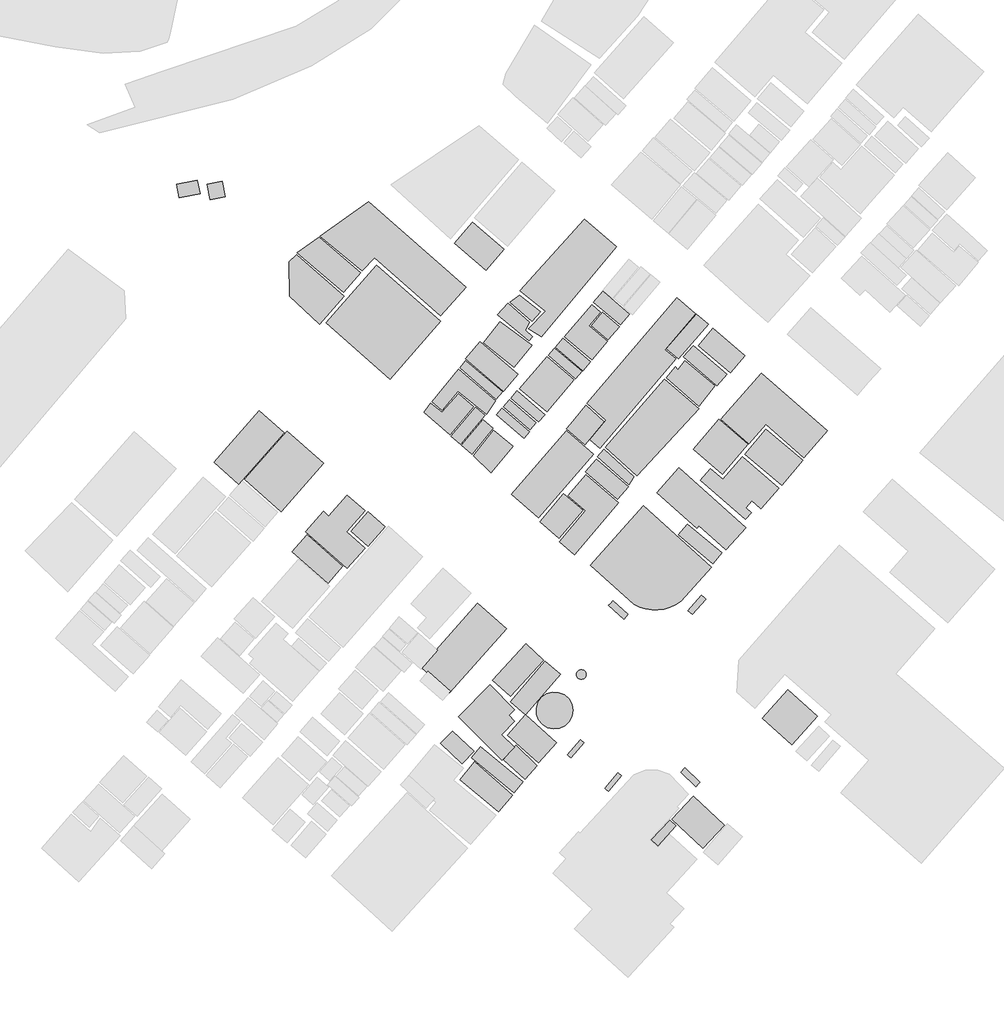
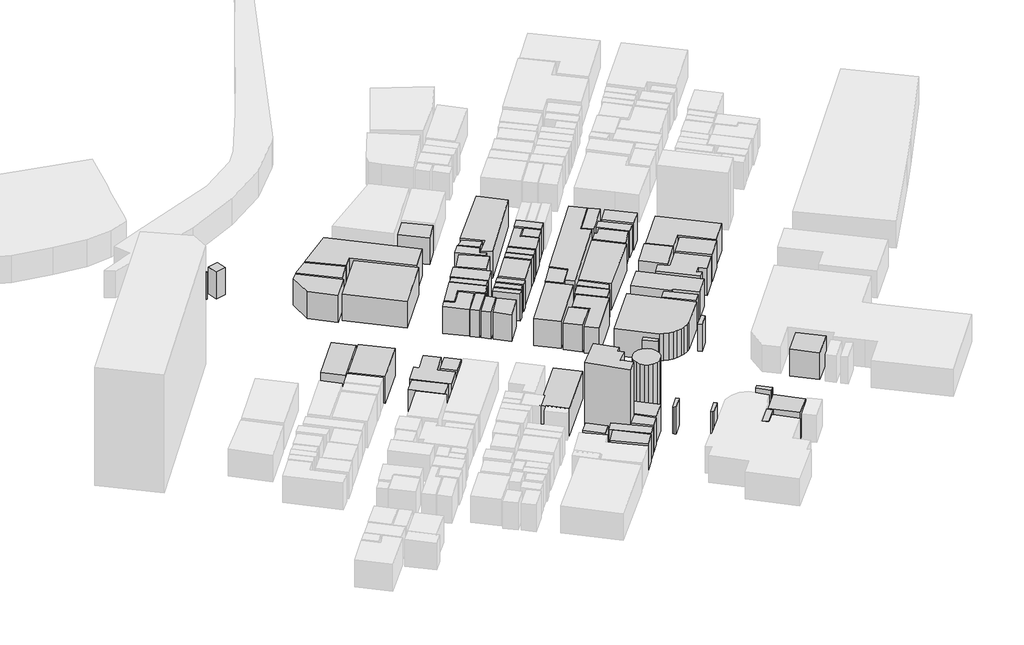
# Not in any storey, part 2 of 3: 70 proxies.
"""IFC4 building model written with IfcOpenShell, lengths in millimetres."""

from ifc_helpers import new_model, si_unit, origin, origin_with_axes, place, context, project, spatial, polyline, outline, extrude, element, save

model = new_model("IFC4")

# Units and contexts
model_context = context("Model", 3, world=origin())
ifc_project = project(units=[si_unit("LENGTHUNIT", "METRE", prefix="MILLI")], contexts=[model_context])

# Site, building
site = spatial("IfcSite", under=ifc_project)
building = spatial("IfcBuilding", under=site)

# Proxies
placement = place(None, origin())
element("IfcBuildingElementProxy", 1, Name="Mass", at=placement, inside=building, context=model_context, shape_type="SweptSolid", body=[
    extrude(outline(polyline([(170698.7323915, 46624.0327425), (171096.1893538, 44511.3291361), (170789.0635192, 42387.5060369), (169804.4542245, 40486.0727911), (168268.8250515, 38984.9412821), (166326.7058014, 38073.1428832), (164194.8911837, 37828.5140449), (162099.2090151, 38284.4132439), (160265.4871197, 39385.2430179), (158883.4208628, 41030.9279318), (158097.5400505, 43054.6755966), (158016.2420351, 45234.096159), (158657.593041, 47313.4412879), (159931.2619458, 49070.3211289), (161719.8182773, 50315.7043068), (163815.500446, 50905.0374178), (165983.4475152, 50782.7229987), (167997.8316659, 49959.8805414), (169623.7919691, 48514.3464955), (170698.7323915, 46624.0327425)])), origin_with_axes(), (0.0, 0.0, 1.0), 35000.0),
])
element("IfcBuildingElementProxy", 2, Name="Mass", at=placement, inside=building, context=model_context, shape_type="SweptSolid", body=[
    extrude(outline(polyline([(130374.9168956, 42153.9966913), (141485.6456275, 53473.6402233), (150256.798147, 44678.1215256), (148287.5795602, 42676.6128464), (150310.9968231, 40486.0727911), (145677.0099623, 35793.6468872), (150175.5001316, 31245.7743872), (145848.6391053, 26586.7069609), (130374.9168956, 42153.9966913)])), origin_with_axes(), (0.0, 0.0, 1.0), 45000.0),
])
element("IfcBuildingElementProxy", 3, Name="Mass", at=placement, inside=building, context=model_context, shape_type="SweptSolid", body=[
    extrude(outline(polyline([(208574.5743203, 165836.1135976), (210995.448548, 168927.3325589), (221636.4554144, 160031.7384269), (215927.5281312, 152781.8292102), (204419.3424371, 162933.9260122), (207608.0312501, 166803.5094596), (208574.5743203, 165836.1135976)])), origin_with_axes(), (0.0, 0.0, 1.0), 15000.0),
])
element("IfcBuildingElementProxy", 4, Name="Mass", at=placement, inside=building, context=model_context, shape_type="SweptSolid", body=[
    extrude(outline(polyline([(177934.2557355, 188964.6583397), (180978.4147472, 186362.6970567), (176868.3484279, 181547.9567328), (183462.5207633, 175921.4934444), (177780.6928194, 169283.1563236), (168151.3945845, 177511.5808958), (177934.2557355, 188964.6583397)])), origin_with_axes(), (0.0, 0.0, 1.0), 15000.0),
])
element("IfcBuildingElementProxy", 5, Name="Mass", at=placement, inside=building, context=model_context, shape_type="SweptSolid", body=[
    extrude(outline(polyline([(164809.1428529, 173875.5067947), (167519.0766882, 177044.562204), (177310.970954, 168671.5842278), (174601.0371162, 165502.5288177), (164809.1428529, 173875.5067947)])), origin_with_axes(), (0.0, 0.0, 1.0), 15000.0),
])
element("IfcBuildingElementProxy", 6, Name="Mass", at=placement, inside=building, context=model_context, shape_type="SweptSolid", body=[
    extrude(outline(polyline([(146282.2285192, 152626.1563127), (148432.1093639, 155139.161655), (157980.1095835, 146988.5735315), (155830.2287387, 144475.5681892), (146282.2285192, 152626.1563127)])), origin_with_axes(), (0.0, 0.0, 1.0), 15000.0),
])
element("IfcBuildingElementProxy", 7, Name="Mass", at=placement, inside=building, context=model_context, shape_type="SweptSolid", body=[
    extrude(outline(polyline([(186524.7459996, 209546.839262), (159931.2619458, 177633.895315), (155288.2419727, 180347.0515252), (161286.2288635, 186629.5648806), (152289.2485248, 193979.5495315), (175215.2887854, 219409.8292553), (186524.7459996, 209546.839262)])), origin_with_axes(), (0.0, 0.0, 1.0), 15000.0),
])
element("IfcBuildingElementProxy", 8, Name="Mass", at=placement, inside=building, context=model_context, shape_type="SweptSolid", body=[
    extrude(outline(polyline([(247760.2176028, 51805.7163239), (258292.8271145, 42287.4306033), (249151.3169721, 32168.6922789), (238618.7074578, 41686.9779995), (247760.2176028, 51805.7163239)])), origin_with_axes(), (0.0, 0.0, 1.0), 15000.0),
])
element("IfcBuildingElementProxy", 9, Name="Mass", at=placement, inside=building, context=model_context, shape_type="SweptSolid", body=[
    extrude(outline(polyline([(145125.990084, 182937.8933163), (156489.6459718, 174520.4373689), (150148.4007948, 166681.1950405), (139254.4667699, 175421.116275), (145125.990084, 182937.8933163)])), origin_with_axes(), (0.0, 0.0, 1.0), 15000.0),
])
element("IfcBuildingElementProxy", 10, Name="Mass", at=placement, inside=building, context=model_context, shape_type="SweptSolid", body=[
    extrude(outline(polyline([(139028.6389507, 148000.447364), (142551.5529376, 144864.7504331), (135026.9699836, 135657.8105068), (131350.4930781, 138860.2243936), (139028.6389507, 148000.447364)])), origin_with_axes(), (0.0, 0.0, 1.0), 15000.0),
])
element("IfcBuildingElementProxy", 11, Name="Mass", at=placement, inside=building, context=model_context, shape_type="SweptSolid", body=[
    extrude(outline(polyline([(215792.0314397, 174387.0034569), (221031.2368575, 180524.9634075), (232394.8927479, 170817.6463118), (227155.6873275, 164679.6863612), (215792.0314397, 174387.0034569)])), origin_with_axes(), (0.0, 0.0, 1.0), 15000.0),
])
element("IfcBuildingElementProxy", 12, Name="Mass", at=placement, inside=building, context=model_context, shape_type="SweptSolid", body=[
    extrude(outline(polyline([(203868.3225562, 173008.1863662), (207725.4617171, 169716.8165378), (180707.4213617, 137803.8725908), (177220.6398263, 140939.5695225), (182839.2359819, 147878.1329448), (176109.5669524, 153916.0174618), (208177.117358, 191455.4246972), (214798.3890328, 185795.6029305), (203868.3225562, 173008.1863662)])), origin_with_axes(), (0.0, 0.0, 1.0), 15000.0),
])
element("IfcBuildingElementProxy", 13, Name="Mass", at=placement, inside=building, context=model_context, shape_type="SweptSolid", body=[
    extrude(outline(polyline([(138025.9634289, 175721.3425765), (151422.0696971, 164268.2651325), (146246.0960676, 158219.2611227), (132849.9898021, 169672.3385674), (138025.9634289, 175721.3425765)])), origin_with_axes(), (0.0, 0.0, 1.0), 15000.0),
])
element("IfcBuildingElementProxy", 14, Name="Mass", at=placement, inside=building, context=model_context, shape_type="SweptSolid", body=[
    extrude(outline(polyline([(162334.0699465, 170951.0802238), (164502.0170183, 173486.3245509), (174230.6794932, 165180.0635306), (172053.6993091, 162633.6997107), (162334.0699465, 170951.0802238)])), origin_with_axes(), (0.0, 0.0, 1.0), 15000.0),
])
element("IfcBuildingElementProxy", 15, Name="Mass", at=placement, inside=building, context=model_context, shape_type="SweptSolid", body=[
    extrude(outline(polyline([(187355.7923757, 118344.7604281), (171556.8781069, 99930.8805755), (166218.3084467, 104512.1115531), (175630.8119747, 115475.9313204), (169334.732359, 120880.0047552), (175721.1431024, 128318.9453478), (187355.7923757, 118344.7604281)])), origin_with_axes(), (0.0, 0.0, 1.0), 15000.0),
])
element("IfcBuildingElementProxy", 16, Name="Mass", at=placement, inside=building, context=model_context, shape_type="SweptSolid", body=[
    extrude(outline(polyline([(168792.745593, 144742.4360131), (170156.7456229, 146410.3599133), (175648.8781992, 153137.6529749), (182152.7194095, 147299.9193266), (175323.6861401, 139104.8532327), (168792.745593, 144742.4360131)])), origin_with_axes(), (0.0, 0.0, 1.0), 15000.0),
])
element("IfcBuildingElementProxy", 17, Name="Mass", at=placement, inside=building, context=model_context, shape_type="SweptSolid", body=[
    extrude(outline(polyline([(144186.5463531, 185328.5842386), (147953.3543863, 189565.1109435), (155676.6658227, 182782.2204187), (154159.1028717, 179813.3158774), (156715.4737935, 177600.5368366), (155333.4075365, 176043.8078635), (144186.5463531, 185328.5842386)])), origin_with_axes(), (0.0, 0.0, 1.0), 15000.0),
])
element("IfcBuildingElementProxy", 18, Name="Mass", at=placement, inside=building, context=model_context, shape_type="SweptSolid", body=[
    extrude(outline(polyline([(148956.0299055, 155661.77781), (151160.1094263, 158241.5001083), (161060.4010443, 149779.5661905), (158856.3215234, 147199.8438922), (148956.0299055, 155661.77781)])), origin_with_axes(), (0.0, 0.0, 1.0), 15000.0),
])
element("IfcBuildingElementProxy", 19, Name="Mass", at=placement, inside=building, context=model_context, shape_type="SweptSolid", body=[
    extrude(outline(polyline([(182649.5406117, 138148.5768635), (203660.5609616, 162455.7878276), (216017.8592589, 151903.3892898), (193940.9315989, 128085.4360023), (182649.5406117, 138148.5768635)])), origin_with_axes(), (0.0, 0.0, 1.0), 15000.0),
])
element("IfcBuildingElementProxy", 20, Name="Mass", at=placement, inside=building, context=model_context, shape_type="SweptSolid", body=[
    extrude(outline(polyline([(143852.3211792, 149790.6856833), (145812.5066538, 152081.3011721), (155622.4671441, 143697.2037031), (153662.2816695, 141395.4687215), (143852.3211792, 149790.6856833)])), origin_with_axes(), (0.0, 0.0, 1.0), 15000.0),
])
element("IfcBuildingElementProxy", 21, Name="Mass", at=placement, inside=building, context=model_context, shape_type="SweptSolid", body=[
    extrude(outline(polyline([(130230.3870919, 157296.3432318), (135695.4203289, 152537.2003711), (127195.2611949, 142629.7324075), (117945.3536977, 150635.7671254), (120375.2610377, 153838.1810131), (124494.3604693, 150591.289155), (130230.3870919, 157296.3432318)])), origin_with_axes(), (0.0, 0.0, 1.0), 15000.0),
])
element("IfcBuildingElementProxy", 22, Name="Mass", at=placement, inside=building, context=model_context, shape_type="SweptSolid", body=[
    extrude(outline(polyline([(120881.1153548, 154405.2751393), (130338.7844466, 166025.1449735), (143545.1953446, 154672.1429632), (140257.1422891, 150001.956044), (130149.0890765, 158152.5441667), (124367.8968926, 151447.4900899), (120881.1153548, 154405.2751393)])), origin_with_axes(), (0.0, 0.0, 1.0), 15000.0),
])
element("IfcBuildingElementProxy", 23, Name="Mass", at=placement, inside=building, context=model_context, shape_type="SweptSolid", body=[
    extrude(outline(polyline([(177654.2292402, 181525.7177472), (181682.9975441, 186251.5021295), (187644.8519858, 181158.7744897), (183607.0505671, 176444.1096002), (177654.2292402, 181525.7177472)])), origin_with_axes(), (0.0, 0.0, 1.0), 15000.0),
])
element("IfcBuildingElementProxy", 24, Name="Mass", at=placement, inside=building, context=model_context, shape_type="SweptSolid", body=[
    extrude(outline(polyline([(142849.64566, 144219.8198581), (149778.0431693, 138471.0421506), (141955.3674929, 129052.8318643), (135659.2878798, 135157.4333365), (142849.64566, 144219.8198581)])), origin_with_axes(), (0.0, 0.0, 1.0), 15000.0),
])
element("IfcBuildingElementProxy", 25, Name="Mass", at=placement, inside=building, context=model_context, shape_type="SweptSolid", body=[
    extrude(outline(polyline([(231563.8463692, 134768.2510935), (244463.1314351, 123582.0414727), (238121.8862556, 116276.5347921), (234933.1974401, 119034.1689735), (232765.2503708, 116532.283124), (234617.0384932, 114919.9566878), (232530.3894394, 112518.1462718), (216550.8129127, 126384.1536245), (220164.0580298, 130542.8438806), (224581.2501837, 126717.7384044), (231563.8463692, 134768.2510935)])), origin_with_axes(), (0.0, 0.0, 1.0), 15000.0),
])
element("IfcBuildingElementProxy", 26, Name="Mass", at=placement, inside=building, context=model_context, shape_type="SweptSolid", body=[
    extrude(outline(polyline([(192902.1236281, 82150.8118051), (177265.8053902, 96139.1335769), (196163.0773468, 117277.2891325), (220516.3494282, 95494.2030027), (209559.183615, 83240.5220863), (207707.3954926, 82039.6168787), (205693.0113393, 81116.6989878), (203579.2629461, 80505.1268912), (201393.2496524, 80193.7810962), (199180.1370193, 80216.0200818), (197003.1568352, 80549.6048616), (194889.4084421, 81205.6549286), (192902.1236281, 82150.8118051)])), origin_with_axes(), (0.0, 0.0, 1.0), 15000.0),
])
element("IfcBuildingElementProxy", 27, Name="Mass", at=placement, inside=building, context=model_context, shape_type="SweptSolid", body=[
    extrude(outline(polyline([(200959.6602385, 121969.7150364), (208881.7001549, 130854.1896757), (232729.1179192, 109571.4807161), (225656.1906061, 101654.4019389), (216053.9917105, 110216.4112902), (215204.8791073, 109260.134921), (200959.6602385, 121969.7150364)])), origin_with_axes(), (0.0, 0.0, 1.0), 15000.0),
])
element("IfcBuildingElementProxy", 28, Name="Mass", at=placement, inside=building, context=model_context, shape_type="SweptSolid", body=[
    extrude(outline(polyline([(175567.5801838, 129464.2530922), (179424.7193472, 133923.1696506), (190842.5739136, 124060.1796573), (186994.4678651, 119601.2630989), (175567.5801838, 129464.2530922)])), origin_with_axes(), (0.0, 0.0, 1.0), 15000.0),
])
element("IfcBuildingElementProxy", 29, Name="Mass", at=placement, inside=building, context=model_context, shape_type="SweptSolid", body=[
    extrude(outline(polyline([(161204.930848, 61913.3351563), (166579.6329599, 57298.7457003), (154249.4340019, 42943.4806703), (148874.73189, 47558.0701262), (161204.930848, 61913.3351563)])), origin_with_axes(), (0.0, 0.0, 1.0), 15000.0),
])
element("IfcBuildingElementProxy", 30, Name="Mass", at=placement, inside=building, context=model_context, shape_type="SweptSolid", body=[
    extrude(outline(polyline([(130916.9036642, 19659.2630314), (135975.4468267, 26086.3297907), (149488.9835592, 14199.5921325), (144493.6721877, 8317.380513), (130916.9036642, 19659.2630314)])), origin_with_axes(), (0.0, 0.0, 1.0), 15000.0),
])
element("IfcBuildingElementProxy", 31, Name="Mass", at=placement, inside=building, context=model_context, shape_type="SweptSolid", body=[
    extrude(outline(polyline([(116861.3801631, 59822.8705346), (137149.751489, 82651.1889753), (147465.5662963, 73488.7270194), (127177.1949678, 50660.4085795), (116861.3801631, 59822.8705346)])), origin_with_axes(), (0.0, 0.0, 1.0), 15000.0),
])
element("IfcBuildingElementProxy", 32, Name="Mass", at=placement, inside=building, context=model_context, shape_type="SweptSolid", body=[
    extrude(outline(polyline([(123961.4068155, 32624.5914779), (128098.5724742, 37050.149558), (135749.6190075, 29889.1962821), (131621.4864611, 25463.6382021), (123961.4068155, 32624.5914779)])), origin_with_axes(), (0.0, 0.0, 1.0), 15000.0),
])
element("IfcBuildingElementProxy", 33, Name="Mass", at=placement, inside=building, context=model_context, shape_type="SweptSolid", body=[
    extrude(outline(polyline([(69220.7433079, 143930.7130486), (82255.5250653, 132444.2771263), (67134.094254, 115275.7804524), (54099.3124992, 126762.2163747), (69220.7433079, 143930.7130486)])), origin_with_axes(), (0.0, 0.0, 1.0), 15000.0),
])
element("IfcBuildingElementProxy", 34, Name="Mass", at=placement, inside=building, context=model_context, shape_type="SweptSolid", body=[
    extrude(outline(polyline([(40612.8751034, 231952.6169812), (45987.5772127, 232975.6103056), (47044.451408, 227426.983466), (41678.7824109, 226403.9901416), (40612.8751034, 231952.6169812)])), origin_with_axes(), (0.0, 0.0, 1.0), 15000.0),
])
element("IfcBuildingElementProxy", 35, Name="Mass", at=placement, inside=building, context=model_context, shape_type="SweptSolid", body=[
    extrude(outline(polyline([(29809.2722061, 231885.9000252), (37198.3584687, 233353.6730567), (38155.868424, 228538.9327328), (30766.7821615, 227071.1597013), (29809.2722061, 231885.9000252)])), origin_with_axes(), (0.0, 0.0, 1.0), 15000.0),
])
element("IfcBuildingElementProxy", 36, Name="Mass", at=placement, inside=building, context=model_context, shape_type="SweptSolid", body=[
    extrude(outline(polyline([(213976.3757689, 13832.6488751), (225105.1707253, 3547.1181603), (217481.2235313, -4703.5453967), (206352.4285723, 5581.985318), (213976.3757689, 13832.6488751)])), origin_with_axes(), (0.0, 0.0, 1.0), 15000.0),
])
element("IfcBuildingElementProxy", 37, Name="Mass", at=placement, inside=building, context=model_context, shape_type="SweptSolid", body=[
    extrude(outline(polyline([(199125.9383406, -1756.879841), (205584.6139871, 5292.8785085), (207788.693508, 3269.1308436), (201339.0509737, -3780.6275059), (199125.9383406, -1756.879841)])), origin_with_axes(), (0.0, 0.0, 1.0), 15000.0),
])
element("IfcBuildingElementProxy", 38, Name="Mass", at=placement, inside=building, context=model_context, shape_type="SweptSolid", body=[
    extrude(outline(polyline([(90367.2603492, 108081.468699), (96970.4657995, 102265.9740355), (90647.286847, 95082.781774), (75823.9487581, 108137.0661622), (82156.1608228, 115320.2584236), (84053.114509, 113652.3345234), (90593.088171, 121080.1556232), (96907.2340111, 115509.2897988), (90367.2603492, 108081.468699)])), origin_with_axes(), (0.0, 0.0, 1.0), 15000.0),
])
element("IfcBuildingElementProxy", 39, Name="Mass", at=placement, inside=building, context=model_context, shape_type="SweptSolid", body=[
    extrude(outline(polyline([(216442.4155605, 18847.5400669), (215647.5016334, 18035.8171024), (214861.6208211, 17224.0941378), (209514.0180486, 22416.897212), (211094.8127879, 24040.343141), (216442.4155605, 18847.5400669)])), origin_with_axes(), (0.0, 0.0, 1.0), 15000.0),
])
element("IfcBuildingElementProxy", 40, Name="Mass", at=placement, inside=building, context=model_context, shape_type="SweptSolid", body=[
    extrude(outline(polyline([(174944.2954023, 58722.0407614), (175404.9841555, 58343.9780104), (175712.1099901, 57821.3618554), (175811.47423, 57220.9092516), (175712.1099901, 56631.5761406), (175414.0172678, 56097.8404928), (174962.3616268, 55708.6582489), (174393.2755215, 55497.3878882), (173842.2556432, 55475.1489034), (173318.3350991, 55630.8218001), (172857.6463485, 55942.1675952), (172523.4211746, 56386.9473015), (172342.7589192, 56909.5634573), (172333.725807, 57454.4185979), (172496.3218352, 57988.1542457), (172812.4807847, 58432.9339519), (173255.1033108, 58766.5187318), (173779.0238523, 58944.4306142), (174375.209297, 58933.3111222), (174944.2954023, 58722.0407614)])), origin_with_axes(), (0.0, 0.0, 1.0), 15000.0),
])
element("IfcBuildingElementProxy", 41, Name="Mass", at=placement, inside=building, context=model_context, shape_type="SweptSolid", body=[
    extrude(outline(polyline([(213642.150595, 78648.1716159), (212151.6869832, 79971.3912426), (216939.2367627, 85353.2256927), (217725.117575, 84663.8171474), (218429.7003744, 84041.125558), (213642.150595, 78648.1716159)])), origin_with_axes(), (0.0, 0.0, 1.0), 15000.0),
])
element("IfcBuildingElementProxy", 42, Name="Mass", at=placement, inside=building, context=model_context, shape_type="SweptSolid", body=[
    extrude(outline(polyline([(223126.9190236, 148089.4033055), (233424.6676038, 139227.1676519), (224310.2568007, 128630.2911429), (214003.4751057, 137492.5267965), (223126.9190236, 148089.4033055)])), origin_with_axes(), (0.0, 0.0, 1.0), 15000.0),
])
element("IfcBuildingElementProxy", 43, Name="Mass", at=placement, inside=building, context=model_context, shape_type="SweptSolid", body=[
    extrude(outline(polyline([(146264.1622947, 26875.8137704), (150753.6193518, 32024.1388742), (158260.1360788, 24640.7957448), (154077.8048588, 19859.4138993), (146264.1622947, 26875.8137704)])), origin_with_axes(), (0.0, 0.0, 1.0), 15000.0),
])
element("IfcBuildingElementProxy", 44, Name="Mass", at=placement, inside=building, context=model_context, shape_type="SweptSolid", body=[
    extrude(outline(polyline([(187066.7327657, 22172.2683729), (188340.4016705, 21082.5580917), (183688.3485825, 15634.0066864), (183056.0306888, 16178.861827), (182414.6796803, 16723.7169676), (187066.7327657, 22172.2683729)])), origin_with_axes(), (0.0, 0.0, 1.0), 15000.0),
])
element("IfcBuildingElementProxy", 45, Name="Mass", at=placement, inside=building, context=model_context, shape_type="SweptSolid", body=[
    extrude(outline(polyline([(185296.2426587, 83418.4339686), (190761.2758982, 78603.6936455), (189288.8785136, 76935.7697453), (183778.6797102, 81828.346518), (184573.5936373, 82662.3084681), (185296.2426587, 83418.4339686)])), origin_with_axes(), (0.0, 0.0, 1.0), 15000.0),
])
element("IfcBuildingElementProxy", 46, Name="Mass", at=placement, inside=building, context=model_context, shape_type="SweptSolid", body=[
    extrude(outline(polyline([(173760.9576278, 33981.1695831), (175034.62653, 32902.5787946), (170382.5734446, 27454.0273886), (169623.7919691, 28098.9579636), (169117.9376521, 28532.618177), (173760.9576278, 33981.1695831)])), origin_with_axes(), (0.0, 0.0, 1.0), 15000.0),
])
element("IfcBuildingElementProxy", 47, Name="Mass", at=placement, inside=building, context=model_context, shape_type="SweptSolid", body=[
    extrude(outline(polyline([(158865.3546357, 25697.1475476), (147727.5265671, 35537.8985561), (154141.0366472, 42798.9272655), (165278.8647184, 32947.056765), (158865.3546357, 25697.1475476)])), origin_with_axes(), (0.0, 0.0, 1.0), 15000.0),
])
element("IfcBuildingElementProxy", 48, Name="Mass", at=placement, inside=building, context=model_context, shape_type="SweptSolid", body=[
    extrude(outline(polyline([(211844.5611486, 110716.7884605), (224165.7269944, 100497.9747017), (221004.1375182, 96683.9887175), (208692.0047847, 106913.921969), (211844.5611486, 110716.7884605)])), origin_with_axes(), (0.0, 0.0, 1.0), 15000.0),
])
element("IfcBuildingElementProxy", 49, Name="Mass", at=placement, inside=building, context=model_context, shape_type="SweptSolid", body=[
    extrude(outline(polyline([(142470.2549222, 55230.5200643), (154339.7651296, 68106.8925701), (160644.8778549, 62302.5173993), (148775.3676501, 49415.0254008), (142470.2549222, 55230.5200643)])), origin_with_axes(), (0.0, 0.0, 1.0), 15000.0),
])
element("IfcBuildingElementProxy", 50, Name="Mass", at=placement, inside=building, context=model_context, shape_type="SweptSolid", body=[
    extrude(outline(polyline([(138071.1289928, 31434.8057624), (153264.8247072, 18925.3765148), (150040.0034401, 15011.315097), (134846.3077282, 27520.7443446), (138071.1289928, 31434.8057624)])), origin_with_axes(), (0.0, 0.0, 1.0), 15000.0),
])
element("IfcBuildingElementProxy", 51, Name="Mass", at=placement, inside=building, context=model_context, shape_type="SweptSolid", body=[
    extrude(outline(polyline([(239829.1445717, 144520.0461604), (252972.3236813, 133467.2704515), (245610.3367581, 124716.2297251), (232467.1576485, 135769.0054331), (239829.1445717, 144520.0461604)])), origin_with_axes(), (0.0, 0.0, 1.0), 15000.0),
])
element("IfcBuildingElementProxy", 52, Name="Mass", at=placement, inside=building, context=model_context, shape_type="SweptSolid", body=[
    extrude(outline(polyline([(98189.9360256, 225692.3426106), (132922.2547027, 195247.1716951), (123916.2412517, 184972.7604732), (100312.717531, 205766.2117561), (95895.5253771, 201051.5468666), (80972.8230482, 213349.7057534), (98189.9360256, 225692.3426106)])), origin_with_axes(), (0.0, 0.0, 1.0), 15000.0),
])
element("IfcBuildingElementProxy", 53, Name="Mass", at=placement, inside=building, context=model_context, shape_type="SweptSolid", body=[
    extrude(outline(polyline([(204491.6073377, 173230.5762197), (215096.4817551, 185639.9300337), (219305.9123144, 182037.2144102), (208692.0047847, 169627.8605962), (204491.6073377, 173230.5762197)])), origin_with_axes(), (0.0, 0.0, 1.0), 15000.0),
])
element("IfcBuildingElementProxy", 54, Name="Mass", at=placement, inside=building, context=model_context, shape_type="SweptSolid", body=[
    extrude(outline(polyline([(132877.0891388, 168949.5715437), (146011.2351362, 157930.1543132), (143680.6920361, 155216.9981038), (130745.2745212, 166481.0441726), (132877.0891388, 168949.5715437)])), origin_with_axes(), (0.0, 0.0, 1.0), 15000.0),
])
element("IfcBuildingElementProxy", 55, Name="Mass", at=placement, inside=building, context=model_context, shape_type="SweptSolid", body=[
    extrude(outline(polyline([(127556.5857056, 142184.9527004), (136354.8375645, 152470.4834152), (139742.2548598, 149579.4153226), (130953.0361158, 139293.8846079), (127556.5857056, 142184.9527004)])), origin_with_axes(), (0.0, 0.0, 1.0), 15000.0),
])
element("IfcBuildingElementProxy", 56, Name="Mass", at=placement, inside=building, context=model_context, shape_type="SweptSolid", body=[
    extrude(outline(polyline([(159262.811598, 111717.5428001), (167799.103186, 121602.771779), (174655.2357922, 115676.0821883), (166118.9442067, 105790.8532102), (159262.811598, 111717.5428001)])), origin_with_axes(), (0.0, 0.0, 1.0), 15000.0),
])
element("IfcBuildingElementProxy", 57, Name="Mass", at=placement, inside=building, context=model_context, shape_type="SweptSolid", body=[
    extrude(outline(polyline([(92011.2868769, 108203.7831182), (98099.6048979, 115108.9880629), (104088.558679, 109827.2290472), (98000.240658, 102922.0241024), (92011.2868769, 108203.7831182)])), origin_with_axes(), (0.0, 0.0, 1.0), 15000.0),
])
element("IfcBuildingElementProxy", 58, Name="Mass", at=placement, inside=building, context=model_context, shape_type="SweptSolid", body=[
    extrude(outline(polyline([(43115.0473466, 132766.7424142), (59284.3192409, 151125.0248028), (68046.4386456, 143408.0968936), (51877.1667513, 125049.8145049), (43115.0473466, 132766.7424142)])), origin_with_axes(), (0.0, 0.0, 1.0), 15000.0),
])
element("IfcBuildingElementProxy", 59, Name="Mass", at=placement, inside=building, context=model_context, shape_type="SweptSolid", body=[
    extrude(outline(polyline([(80602.4654227, 213005.0014807), (95326.4392717, 200428.8552772), (89301.3530417, 193367.977435), (72788.8228612, 207467.4941339), (80602.4654227, 213005.0014807)])), origin_with_axes(), (0.0, 0.0, 1.0), 15000.0),
])
element("IfcBuildingElementProxy", 60, Name="Mass", at=placement, inside=building, context=model_context, shape_type="SweptSolid", body=[
    extrude(outline(polyline([(128902.519511, 210814.4614255), (135343.1289304, 218320.118974), (146535.1556777, 208723.9968047), (140094.5462583, 201218.3392562), (128902.519511, 210814.4614255)])), origin_with_axes(), (0.0, 0.0, 1.0), 15000.0),
])
element("IfcBuildingElementProxy", 61, Name="Mass", at=placement, inside=building, context=model_context, shape_type="SweptSolid", body=[
    extrude(outline(polyline([(210552.8260193, 170361.7471128), (213958.3095418, 174353.6449785), (225900.0846498, 164157.0702054), (222485.5680151, 160165.1723388), (210552.8260193, 170361.7471128)])), origin_with_axes(), (0.0, 0.0, 1.0), 15000.0),
])
element("IfcBuildingElementProxy", 62, Name="Mass", at=placement, inside=building, context=model_context, shape_type="SweptSolid", body=[
    extrude(outline(polyline([(148712.1358592, 189787.500797), (152072.4538178, 192344.9841097), (159461.5400804, 186485.0114758), (156489.6459718, 183149.1636762), (148712.1358592, 189787.500797)])), origin_with_axes(), (0.0, 0.0, 1.0), 15000.0),
])
element("IfcBuildingElementProxy", 63, Name="Mass", at=placement, inside=building, context=model_context, shape_type="SweptSolid", body=[
    extrude(outline(polyline([(149172.8246124, 121358.1429399), (168702.4144653, 143975.1910198), (178340.7458125, 135668.9299996), (158811.1559596, 113051.8819196), (149172.8246124, 121358.1429399)])), origin_with_axes(), (0.0, 0.0, 1.0), 15000.0),
])
element("IfcBuildingElementProxy", 64, Name="Mass", at=placement, inside=building, context=model_context, shape_type="SweptSolid", body=[
    extrude(outline(polyline([(101035.366555, 203019.6970675), (123834.9432363, 183026.849257), (105831.9494467, 162489.146306), (83032.3727653, 182470.8746236), (101035.366555, 203019.6970675)])), origin_with_axes(), (0.0, 0.0, 1.0), 15000.0),
])
element("IfcBuildingElementProxy", 65, Name="Mass", at=placement, inside=building, context=model_context, shape_type="SweptSolid", body=[
    extrude(outline(polyline([(72544.9288149, 206811.4440662), (89482.015297, 192055.877301), (80801.1939052, 182081.6923806), (70133.0876994, 191944.6823739), (69889.1936557, 204365.1556806), (72544.9288149, 206811.4440662)])), origin_with_axes(), (0.0, 0.0, 1.0), 15000.0),
])
element("IfcBuildingElementProxy", 66, Name="Mass", at=placement, inside=building, context=model_context, shape_type="SweptSolid", body=[
    extrude(outline(polyline([(178476.2425041, 189898.6957242), (181728.1631079, 193701.5622148), (191221.9646488, 185595.4520625), (187970.0440449, 181781.4660791), (178476.2425041, 189898.6957242)])), origin_with_axes(), (0.0, 0.0, 1.0), 15000.0),
])
element("IfcBuildingElementProxy", 67, Name="Mass", at=placement, inside=building, context=model_context, shape_type="SweptSolid", body=[
    extrude(outline(polyline([(152072.4538178, 159086.5815504), (161774.016956, 170428.4640687), (171439.4476399, 162166.6810189), (161746.9176166, 150824.7985005), (152072.4538178, 159086.5815504)])), origin_with_axes(), (0.0, 0.0, 1.0), 15000.0),
])
element("IfcBuildingElementProxy", 68, Name="Mass", at=placement, inside=building, context=model_context, shape_type="SweptSolid", body=[
    extrude(outline(polyline([(182179.8187463, 137503.6462893), (192911.156743, 127729.6122368), (191068.4017328, 124738.4687099), (179758.9445185, 134790.4900791), (182179.8187463, 137503.6462893)])), origin_with_axes(), (0.0, 0.0, 1.0), 15000.0),
])
element("IfcBuildingElementProxy", 69, Name="Mass", at=placement, inside=building, context=model_context, shape_type="SweptSolid", body=[
    extrude(outline(polyline([(238356.747187, 164635.20839), (261779.6086524, 144053.0274686), (253378.8137584, 134490.2637768), (239883.3432503, 146354.7624501), (233840.1907932, 139471.7964902), (223912.7998359, 148200.5982319), (238356.747187, 164635.20839)])), origin_with_axes(), (0.0, 0.0, 1.0), 15000.0),
])
element("IfcBuildingElementProxy", 70, Name="Mass", at=placement, inside=building, context=model_context, shape_type="SweptSolid", body=[
    extrude(outline(polyline([(76257.538172, 106925.0414618), (88994.2272071, 95705.4733634), (83782.121126, 89801.0227583), (71054.4652058, 101009.4713639), (76257.538172, 106925.0414618)])), origin_with_axes(), (0.0, 0.0, 1.0), 15000.0),
])

save(model, "model.ifc")

# Revit data of these elements
# Elements 1, 2, 3, 4, 5, 6, 7, 8, 9, 10, 11, 12, 13, 14, 15, 16, 17, 18, 19, 20, 21, 22, 23, 24, 25, 26, 27, 28, 29, 30, 31, 32, 33, 34, 35, 36, 37, 38, 39, 40, 41, 42, 43, 44, 45, 46, 47, 48, 49, 50, 51, 52, 53, 54, 55, 56, 57, 58, 59, 60, 61, 62, 63, 64, 65, 66, 67, 68, 69, 70 (IfcBuildingElementProxy)
#   Phase Created = 新しい建設
#   Materials on its faces: "周辺建物"
# Materials
#   "周辺建物": class "一般", colour RGB 120 120 120, transparency 0, Cost = 0
